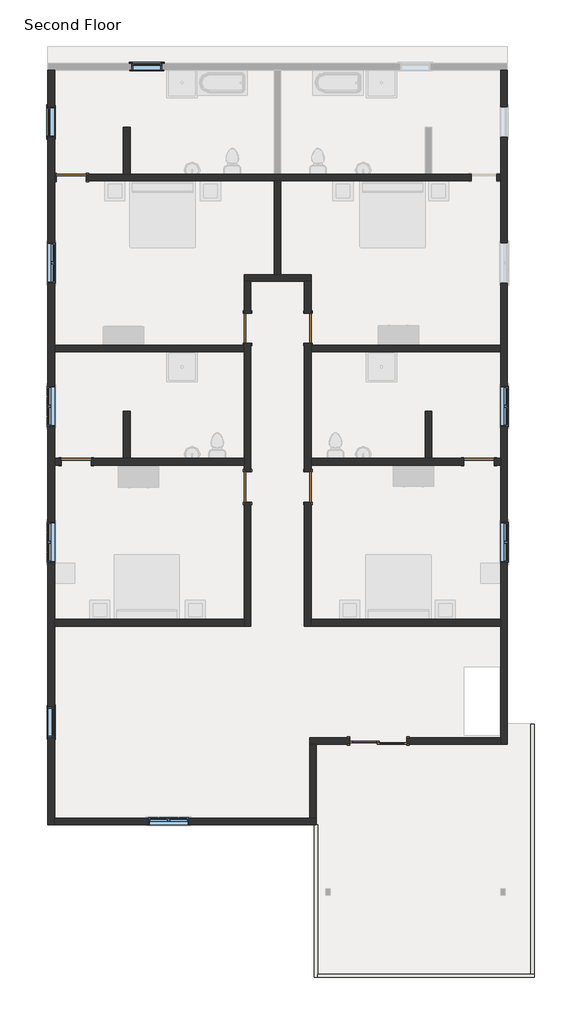
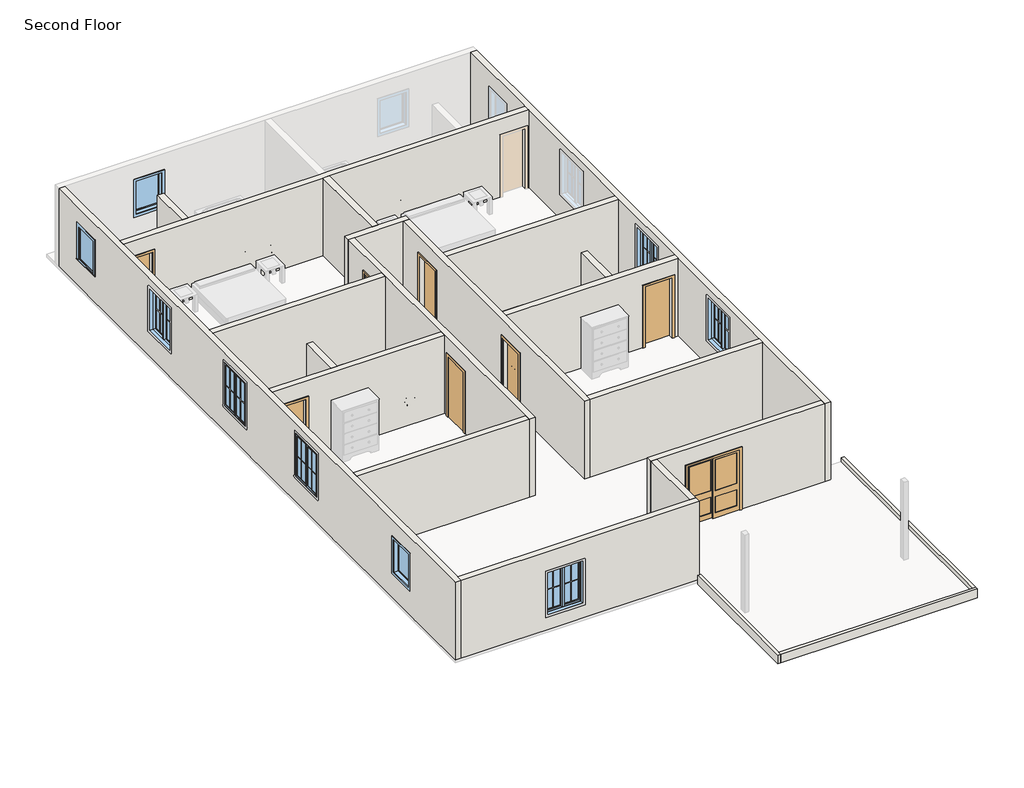
# One storey, part 1 of 2: 22 walls, 9 windows, 8 doors.
# Revit data of these elements (continued)
# Type "Window-Casement-Double : 48\" x 60\"" (continued)
#   Exterior Trim Material = Clad - White
#   Exterior Trim = Trim-Window-Exterior-Flat : with Sill
#   Exterior Frame Material = Clad - White
#   Wall Closure = (empty or 0)
# Elements 1, 2, 3, 4, 5, 6, 7 (IfcDoor, "Single-Flush : 36\" x 84\"")
#   Phase Created = New Construction
#   Materials on its faces: "Door - Frame", "Door - Panel"
# Element 8 (IfcDoor, "Sliding-Closet : 68\" x 84\"")
#   Phase Created = New Construction
#   Materials on its faces: "Door - Panel", "Door - Frame"
# Elements 9, 10, 11 (IfcWall, "Generic - 4\"")
#   built-in parameter 1001111 = -0' - 6"
#   Top Offset = 0' - 0"
#   Base Offset = -0' - 6"
#   Unconnected Height = 1' - 0"
#   wall height = 1' - 0"
#   Phase Created = New Construction
#   Base Constraint = Second Floor
#   Materials on its faces: "Default Wall"
# Elements 12, 13, 14, 15, 16, 17, 18, 19, 20, 21, 22, 23, 24, 25, 26, 27, 28, 29 (IfcWall, "Generic - 8\" - Filled")
#   Top Offset = 0' - 0"
#   Base Offset = 0' - 0"
#   Unconnected Height = 9' - 0"
#   wall height = 9' - 0"
#   Phase Created = New Construction
#   Base Constraint = Second Floor
#   Materials on its faces: "Default Wall"
# Element 30 (IfcWall, "Generic - 8\" - Filled 2")
#   Top Offset = 0' - 0"
#   Base Offset = 0' - 0"
#   Unconnected Height = 9' - 0"
#   wall height = 9' - 0"
#   Phase Created = New Construction
#   Base Constraint = Second Floor
#   Materials on its faces: "Default Wall"
# Element 31 (IfcWindow, "Fixed with Trim : 36\" x 48\"")
#   Mark = "30"
#   Phase Created = New Construction
#   Materials on its faces: "Sash", "Trim", "Glass"
# Element 32 (IfcWindow, "Fixed with Trim : 36\" x 48\"")
#   Mark = "36"
#   Phase Created = New Construction
#   Materials on its faces: "Sash", "Trim", "Glass"
# Element 33 (IfcWindow, "Fixed with Trim : 36\" x 48\"")
#   Mark = "44"
#   Phase Created = New Construction
#   Materials on its faces: "Sash", "Trim", "Glass"
# Element 34 (IfcWindow, "Window-Casement-Double : 48\" x 60\"")
#   Mark = "40"
#   Window Inset = 0' - 0"
#   Interior Wall Closure = 0' - 2 1/4"
#   Frame Extension = 0' - 0 1/4"
#   Exterior Wall Closure = 0' - 1 1/4"
#   Interior Trim Visibility = yes
#   Exterior Trim Visibility = yes
#   Phase Created = New Construction
#   Materials on its faces: "Wood - Stained", "Glass", "Clad - White"
# Element 35 (IfcWindow, "Window-Casement-Double : 48\" x 60\"")
#   Mark = "41"
#   Window Inset = 0' - 0"
#   Interior Wall Closure = 0' - 2 1/4"
#   Frame Extension = 0' - 0 1/4"
#   Exterior Wall Closure = 0' - 1 1/4"
#   Interior Trim Visibility = yes
#   Exterior Trim Visibility = yes
#   Phase Created = New Construction
#   Materials on its faces: "Wood - Stained", "Glass", "Clad - White"
# Element 36 (IfcWindow, "Window-Casement-Double : 48\" x 60\"")
#   Mark = "42"
#   Window Inset = 0' - 0"
#   Interior Wall Closure = 0' - 2 1/4"
#   Frame Extension = 0' - 0 1/4"
#   Exterior Wall Closure = 0' - 1 1/4"
#   Interior Trim Visibility = yes
#   Exterior Trim Visibility = yes
#   Phase Created = New Construction
#   Materials on its faces: "Wood - Stained", "Glass", "Clad - White"
# Element 37 (IfcWindow, "Window-Casement-Double : 48\" x 60\"")
#   Mark = "43"
#   Window Inset = 0' - 0"
#   Interior Wall Closure = 0' - 2 1/4"
#   Frame Extension = 0' - 0 1/4"
#   Exterior Wall Closure = 0' - 1 1/4"
#   Interior Trim Visibility = yes
#   Exterior Trim Visibility = yes
#   Phase Created = New Construction
#   Materials on its faces: "Wood - Stained", "Glass", "Clad - White"
# Element 38 (IfcWindow, "Window-Casement-Double : 48\" x 60\"")
#   Mark = "47"
#   Window Inset = 0' - 0"
#   Interior Wall Closure = 0' - 2 1/4"
#   Frame Extension = 0' - 0 1/4"
#   Exterior Wall Closure = 0' - 1 1/4"
#   Interior Trim Visibility = yes
#   Exterior Trim Visibility = yes
#   Phase Created = New Construction
#   Materials on its faces: "Wood - Stained", "Glass", "Clad - White"
# Element 39 (IfcWindow, "Window-Casement-Double : 48\" x 60\"")
#   Mark = "45"
#   Window Inset = 0' - 0"
#   Interior Wall Closure = 0' - 2 1/4"
#   Frame Extension = 0' - 0 1/4"
#   Exterior Wall Closure = 0' - 1 1/4"
#   Interior Trim Visibility = yes
#   Exterior Trim Visibility = yes
#   Phase Created = New Construction
#   Materials on its faces: "Wood - Stained", "Glass", "Clad - White"
# Materials
#   "Door - Panel": class "Wood", colour RGB 227 170 128, transparency 0, Cost = 0
#   "Door - Frame": class "Miscellaneous", colour RGB 153 76 43, transparency 0, Cost = 0
#   "Glass": class "Glass", colour RGB 236 240 239, transparency 0.5, Description = "Soda Lime Glass", Cost = 0
#   "Sash": class "Wood", colour RGB 227 170 128, transparency 0, Cost = 0
#   "Trim": class "Wood", colour RGB 227 170 128, transparency 0, Cost = 0
#   "Wood - Stained": class "Wood", colour RGB 224 178 126, transparency 0, Cost = 0
#   "Clad - White": class "Wood", colour RGB 216 216 204, transparency 0, Cost = 0
#   "Default Wall": class "Miscellaneous", colour RGB 80 80 80, transparency 0, Cost = 0
# Room at (4233.719, 735.333) mm, phase "New Construction", upper level "Second Floor", upper offset 9' - 0", lower offset 0' - 0"
#   Number = "6"
#   Name = "Room"
# Room at (-3044.815, 735.333) mm, phase "New Construction", upper level "Second Floor", upper offset 9' - 0", lower offset 0' - 0"
#   Number = "7"
#   Name = "Room"
# Room at (-3044.815, -6719.865) mm, phase "New Construction", upper level "Second Floor", upper offset 9' - 0", lower offset 0' - 0"
#   Number = "8"
#   Name = "Room"
# Room at (4233.719, -7666.748) mm, phase "New Construction", upper level "Second Floor", upper offset 9' - 0", lower offset 0' - 0"
#   Number = "9"
#   Name = "Room"
